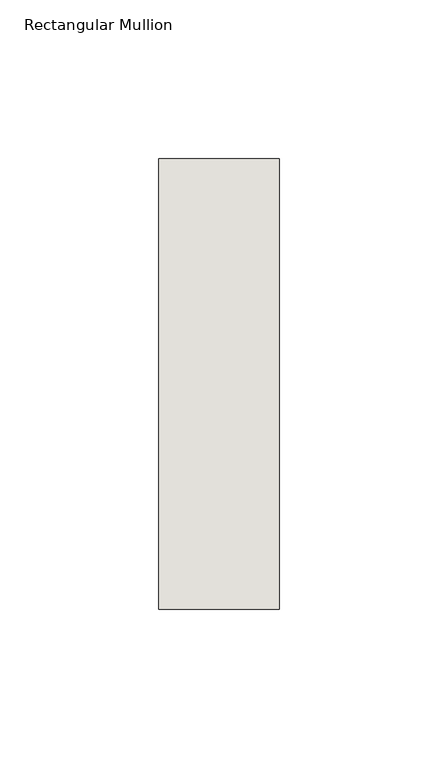
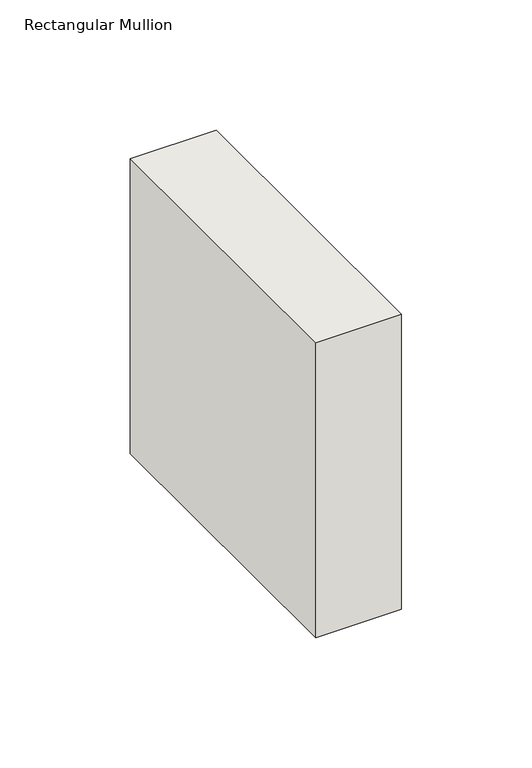
"""IFC4 building model written with IfcOpenShell, lengths in millimetres: wall geometry, Rectangular Mullion : NLRS_21_CWM_hsb-regel 38x142_gen_rsf."""

from ifc_helpers import new_model, si_unit, frame, origin, place, context, project, spatial, polyline, outline, extrude, source, transform, mapped, element, save


def rectangular_mullion_d39b2c0b(model_context):
    return source(origin(), model_context, "Body", "SweptSolid", [
        extrude(outline(polyline([(-38.0, -71.0), (-38.0, 71.0), (0.0, 71.0), (0.0, -71.0), (-38.0, -71.0)])), frame((0.0, 0.0, -137.9999997), z_axis=(0.0, 0.0, 1.0), x_axis=(1.0, 0.0, 0.0)), (0.0, 0.0, 1.0), 137.9999997),
    ])


if __name__ == "__main__":
    model = new_model("IFC4")
    model_context = context("Model", 3, world=origin())
    ifc_project = project(units=[si_unit("LENGTHUNIT", "METRE", prefix="MILLI")], contexts=[model_context])
    site = spatial("IfcSite", under=ifc_project)
    building = spatial("IfcBuilding", under=site)
    placement = place(None, origin())
    rectangular_mullion_shape = rectangular_mullion_d39b2c0b(model_context)
    element("IfcWall", 1, ObjectType="Rectangular Mullion : NLRS_21_CWM_hsb-regel 38x142_gen_rsf", at=placement, inside=building, context=model_context, shape_type="MappedRepresentation", body=[
        mapped(rectangular_mullion_shape, transform((0.0, 0.0, 0.0), x_axis=(1.0, 0.0, 0.0), y_axis=(0.0, 1.0, 0.0), z_axis=(0.0, 0.0, 1.0))),
    ])
    save(model, "model.ifc")

# Revit data of these elements
# Type "Rectangular Mullion : NLRS_21_CWM_hsb-regel 38x142_gen_rsf"
#   Type IfcGUID = "07M7mRoiH1CR8m_RSKIwpF"
#   Assembly Code = "21.10"
#   IfcExportAs = "IfcWall"
#   built-in parameter 1007322 = 0.465879 (stored number, unit not read)
#   built-in parameter 1007321 = 0.062336 (stored number, unit not read)
#   built-in parameter 1007320 = 0.062336 (stored number, unit not read)
# Element 1 (IfcWall, "Rectangular Mullion : NLRS_21_CWM_hsb-regel 38x142_gen_rsf")
#   Materials on its faces: "NLRS_i2_hout naaldhout vuren_gen_rsf"
# Materials
#   "NLRS_i2_hout naaldhout vuren_gen_rsf": class "I - Hout", colour RGB 234 199 147, transparency 0, Keynote = "i2", Manufacturer = "Revit Standards Foundation", URL = "www.revitstandards.org", Description = "hout vuren", Cost = 0
